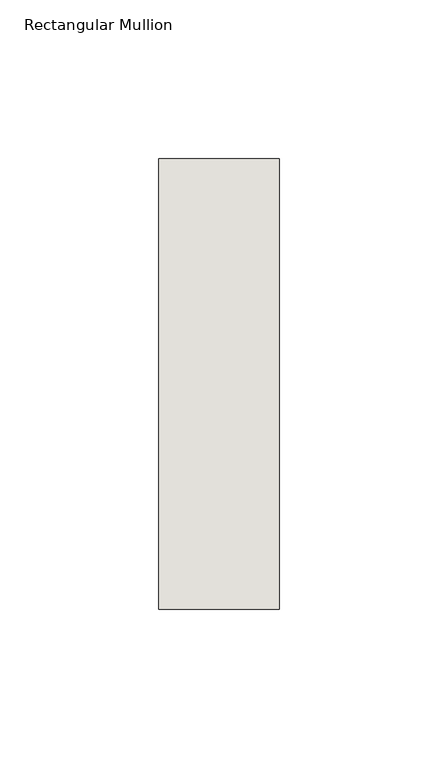
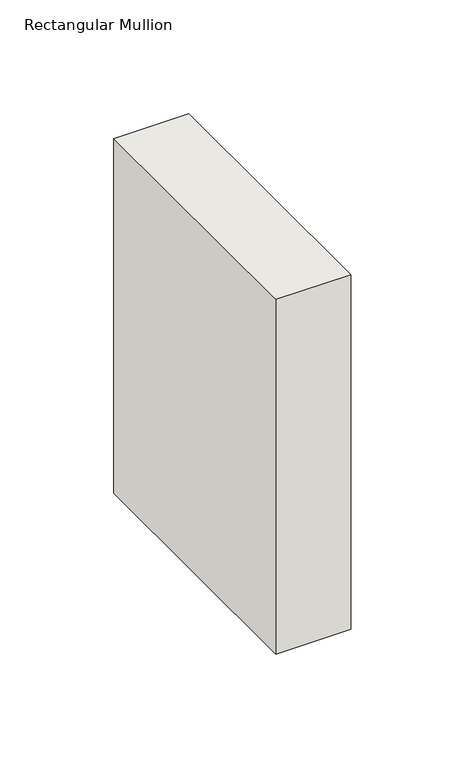
"""IFC4 building model written with IfcOpenShell, lengths in millimetres: wall geometry, Rectangular Mullion : NLRS_21_CWM_hsb-regel 38x142_gen_rsf."""

from ifc_helpers import new_model, si_unit, frame, origin, place, context, project, spatial, polyline, outline, extrude, source, transform, mapped, element, save


def rectangular_mullion_50c5102b(model_context):
    return source(origin(), model_context, "Body", "SweptSolid", [
        extrude(outline(polyline([(0.0, -71.0), (-38.0, -71.0), (-38.0, 71.0), (0.0, 71.0), (0.0, -71.0)])), frame((0.0, 0.0, -189.9999997), z_axis=(0.0, 0.0, 1.0), x_axis=(1.0, 0.0, 0.0)), (0.0, 0.0, 1.0), 189.9999997),
    ])


if __name__ == "__main__":
    model = new_model("IFC4")
    model_context = context("Model", 3, world=origin())
    ifc_project = project(units=[si_unit("LENGTHUNIT", "METRE", prefix="MILLI")], contexts=[model_context])
    site = spatial("IfcSite", under=ifc_project)
    building = spatial("IfcBuilding", under=site)
    placement = place(None, origin())
    rectangular_mullion_shape = rectangular_mullion_50c5102b(model_context)
    element("IfcWall", 1, ObjectType="Rectangular Mullion : NLRS_21_CWM_hsb-regel 38x142_gen_rsf", at=placement, inside=building, context=model_context, shape_type="MappedRepresentation", body=[
        mapped(rectangular_mullion_shape, transform((0.0, 0.0, 0.0), x_axis=(1.0, 0.0, 0.0), y_axis=(0.0, 1.0, 0.0), z_axis=(0.0, 0.0, 1.0))),
    ])
    save(model, "model.ifc")

# Revit data of these elements
# Type "Rectangular Mullion : NLRS_21_CWM_hsb-regel 38x142_gen_rsf"
#   Type IfcGUID = "07M7mRoiH1CR8m_RSKIwpF"
#   Assembly Code = "21.10"
#   IfcExportAs = "IfcWall"
#   built-in parameter 1007322 = 0.465879 (stored number, unit not read)
#   built-in parameter 1007321 = 0.062336 (stored number, unit not read)
#   built-in parameter 1007320 = 0.062336 (stored number, unit not read)
# Element 1 (IfcWall, "Rectangular Mullion : NLRS_21_CWM_hsb-regel 38x142_gen_rsf")
#   Materials on its faces: "NLRS_i2_hout naaldhout vuren_gen_rsf"
# Materials
#   "NLRS_i2_hout naaldhout vuren_gen_rsf": class "I - Hout", colour RGB 234 199 147, transparency 0, Keynote = "i2", Manufacturer = "Revit Standards Foundation", URL = "www.revitstandards.org", Description = "hout vuren", Cost = 0
